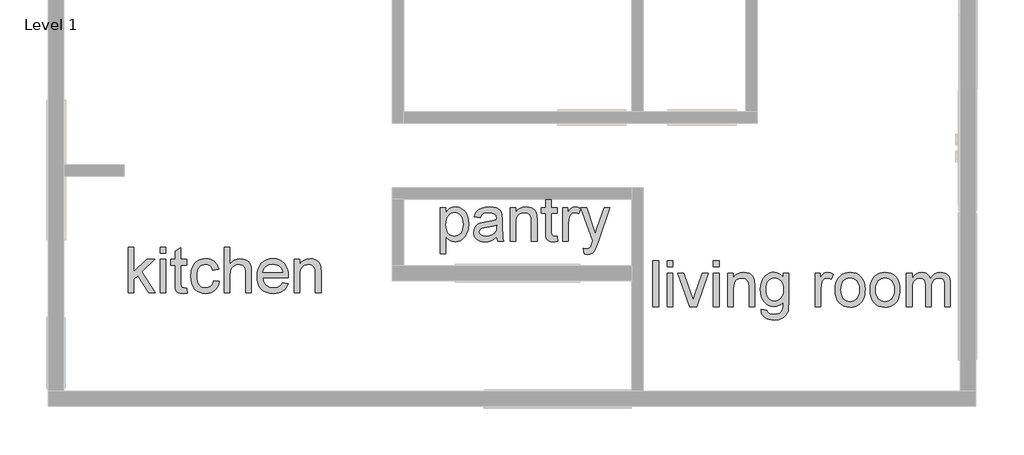
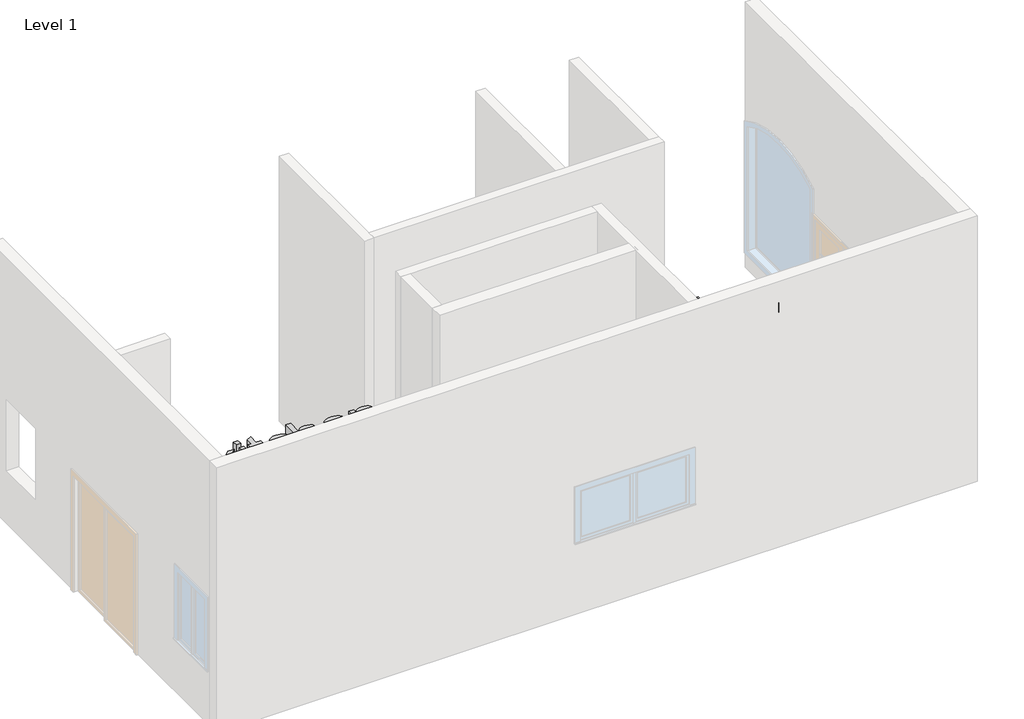
# One storey, part 2 of 3: 3 proxies.
"""IFC4 building model written with IfcOpenShell, lengths in millimetres."""

from ifc_helpers import new_model, si_unit, origin, origin_with_axes, place, context, project, spatial, polyline, outline, extrude, element, save

model = new_model("IFC4")

# Units and contexts
model_context = context("Model", 3, world=origin())
ifc_project = project(units=[si_unit("LENGTHUNIT", "METRE", prefix="MILLI")], contexts=[model_context])

# Site, building, storey
site = spatial("IfcSite", under=ifc_project)
building = spatial("IfcBuilding", under=site)
storey = spatial("IfcBuildingStorey", under=building, Name="Level 1", Elevation=0.0)

# Proxies
placement = place(None, origin())
element("IfcBuildingElementProxy", 1, Name="24\" Arial", ObjectType="24\" Arial", at=placement, inside=storey, context=model_context, shape_type="SweptSolid", body=[
    extrude(outline(polyline([(-77396.9155142, -11295.8130621), (-77396.9155142, -10686.678874), (-77320.7737407, -10686.678874), (-77320.7737407, -11013.9992715), (-77150.0496079, -10848.4801427), (-77044.7598117, -10848.4801427), (-77217.5659461, -11016.0812731), (-77035.24209, -11295.8130621), (-77124.1733021, -11295.8130621), (-77272.1441314, -11069.0236), (-77320.7737407, -11116.1660652), (-77320.7737407, -11295.8130621), (-77396.9155142, -11295.8130621)])), origin_with_axes(), (0.0, 0.0, 1.0), 152.4),
    extrude(outline(polyline([(-76968.6180382, -11295.8130621), (-76968.6180382, -10848.4801427), (-76892.4762647, -10848.4801427), (-76892.4762647, -11295.8130621), (-76968.6180382, -11295.8130621)])), origin_with_axes(), (0.0, 0.0, 1.0), 152.4),
    extrude(outline(polyline([(-76968.6180382, -10762.8206475), (-76968.6180382, -10686.678874), (-76892.4762647, -10686.678874), (-76892.4762647, -10762.8206475), (-76968.6180382, -10762.8206475)])), origin_with_axes(), (0.0, 0.0, 1.0), 152.4),
    extrude(outline(polyline([(-76616.4623357, -11232.3120127), (-76606.944614, -11298.0437781), (-76637.0964589, -11303.5090324), (-76663.9022297, -11305.3307838), (-76700.4487939, -11302.1706028), (-76727.7007079, -11292.6900597), (-76746.9592229, -11278.0788698), (-76759.5255898, -11259.5267482), (-76766.4408095, -11227.6646877), (-76768.7458827, -11173.123681), (-76768.7458827, -10924.6219162), (-76825.8522128, -10924.6219162), (-76825.8522128, -10848.4801427), (-76768.7458827, -10848.4801427), (-76768.7458827, -10739.7699153), (-76692.6041092, -10695.0068805), (-76692.6041092, -10848.4801427), (-76616.4623357, -10848.4801427), (-76616.4623357, -10924.6219162), (-76692.6041092, -10924.6219162), (-76692.6041092, -11170.892965), (-76688.5888204, -11210.1535669), (-76675.5763102, -11224.0583635), (-76664.5900338, -11227.9063486), (-76649.6256472, -11229.1890103), (-76616.4623357, -11232.3120127)])), origin_with_axes(), (0.0, 0.0, 1.0), 152.4),
    extrude(outline(polyline([(-76254.7889115, -11134.0117934), (-76178.6471379, -11143.5295151), (-76186.9286712, -11179.457985), (-76199.8761187, -11211.2503356), (-76217.4894807, -11238.906567), (-76239.7687569, -11262.426679), (-76265.7751879, -11281.1972249), (-76294.5700138, -11294.6047576), (-76326.1532348, -11302.6492773), (-76360.5248509, -11305.3307838), (-76403.2291207, -11301.5896872), (-76441.5184317, -11290.3663972), (-76475.392784, -11271.6609139), (-76504.8521774, -11245.4732373), (-76528.6976022, -11212.2959838), (-76545.7300485, -11172.6217699), (-76555.9495163, -11126.4505956), (-76559.3560055, -11073.7824608), (-76553.5375546, -11006.0244617), (-76546.2644909, -10975.5333621), (-76536.0822017, -10947.3008624), (-76522.9209772, -10921.8939364), (-76506.7111074, -10899.8795577), (-76487.4525925, -10881.2577262), (-76465.1454322, -10866.0284421), (-76440.7980963, -10854.1870579), (-76415.4190543, -10845.7289263), (-76389.0083061, -10840.6540473), (-76361.5658517, -10838.962421), (-76327.7844459, -10841.2860835), (-76297.2282838, -10848.2570711), (-76269.8973652, -10859.8753837), (-76245.7916902, -10876.1410214), (-76225.3202234, -10896.6821981), (-76208.8919293, -10921.1271278), (-76196.5068081, -10949.4758106), (-76188.1648596, -10981.7282464), (-76264.3066332, -10991.2459681), (-76278.1184832, -10958.0268886), (-76299.6263035, -10934.2139951), (-76327.6403789, -10919.8816447), (-76360.9709941, -10915.1041945), (-76386.8426526, -10917.455741), (-76410.1768716, -10924.5103804), (-76430.9736512, -10936.2681128), (-76449.2329913, -10952.7289381), (-76464.0997841, -10974.273937), (-76474.7189218, -11001.2841902), (-76481.0904045, -11033.7596976), (-76483.214232, -11071.7004592), (-76481.1368777, -11110.2128419), (-76474.9048148, -11143.0647826), (-76464.5180434, -11170.2562814), (-76449.9765633, -11191.7873383), (-76432.0797146, -11208.1505698), (-76411.626837, -11219.8385923), (-76388.6179308, -11226.8514058), (-76363.0529957, -11229.1890103), (-76323.62509, -11223.35197), (-76306.5740544, -11216.0556697), (-76291.298297, -11205.8408493), (-76278.2253717, -11192.5959729), (-76267.7828323, -11176.2095048), (-76259.9706789, -11156.681445), (-76254.7889115, -11134.0117934)])), origin_with_axes(), (0.0, 0.0, 1.0), 152.4),
    extrude(outline(polyline([(-76112.0230861, -11295.8130621), (-76112.0230861, -10686.678874), (-76035.8813126, -10686.678874), (-76035.8813126, -10910.6427625), (-76007.9137105, -10879.2826131), (-75976.5070878, -10856.8825064), (-75941.6614447, -10843.4424424), (-75903.376781, -10838.962421), (-75857.3868523, -10843.851407), (-75817.8660002, -10858.5183648), (-75786.7475117, -10881.8107579), (-75775.0641365, -10896.2592915), (-75765.9646741, -10912.5760497), (-75754.253415, -10954.8481183), (-75750.3496619, -11012.6608419), (-75750.3496619, -11295.8130621), (-75826.4914354, -11295.8130621), (-75826.4914354, -11020.5427051), (-75828.0064634, -10994.833703), (-75832.5515473, -10972.8797395), (-75840.1266871, -10954.6808146), (-75850.7318829, -10940.2369284), (-75864.116179, -10929.2413573), (-75880.0286199, -10921.387378), (-75898.4692057, -10916.6749904), (-75919.4379363, -10915.1041945), (-75951.6160149, -10919.342555), (-75981.8236277, -10932.0576363), (-76006.8448257, -10952.0225447), (-76023.4636601, -10978.0103863), (-76032.7768995, -11012.5493061), (-76035.8813126, -11058.1674487), (-76035.8813126, -11295.8130621), (-76112.0230861, -11295.8130621)])), origin_with_axes(), (0.0, 0.0, 1.0), 152.4),
    extrude(outline(polyline([(-75332.462194, -11162.5649585), (-75257.8075645, -11172.0826802), (-75269.2539261, -11201.9835695), (-75284.7062818, -11228.3339025), (-75304.1646318, -11251.1336792), (-75327.6289759, -11270.3828995), (-75354.8576534, -11285.6725989), (-75385.6090032, -11296.5938127), (-75419.8830254, -11303.146541), (-75457.67972, -11305.3307838), (-75504.9244264, -11301.5618032), (-75547.0198966, -11290.2548614), (-75583.9661307, -11271.4099583), (-75615.7631286, -11245.027094), (-75641.332711, -11211.8405459), (-75659.5966985, -11172.5845913), (-75670.5550909, -11127.2592301), (-75674.2078884, -11075.8644625), (-75670.5179123, -11022.7269479), (-75659.4479841, -10975.8912061), (-75640.9981036, -10935.3572371), (-75615.168271, -10901.1250408), (-75583.4549249, -10873.9288947), (-75547.354504, -10854.503076), (-75506.8670082, -10842.8475848), (-75461.9924376, -10838.962421), (-75418.5631851, -10842.8382901), (-75379.2886411, -10854.4658974), (-75344.1688058, -10873.8452428), (-75313.203679, -10900.9763264), (-75287.9268781, -10935.1341655), (-75269.8720203, -10975.5937773), (-75259.0391056, -11022.3551619), (-75255.4281341, -11075.4183193), (-75255.8742773, -11095.9409066), (-75598.0661149, -11095.9409066), (-75593.6558034, -11126.3251178), (-75584.8863011, -11152.935701), (-75571.7576078, -11175.7726562), (-75554.2697237, -11194.8359836), (-75533.3892922, -11209.8654328), (-75510.0829572, -11220.6007536), (-75484.3507184, -11227.0419461), (-75456.1925759, -11229.1890103), (-75415.6679016, -11225.2109001), (-75381.5379464, -11213.2765694), (-75353.8027106, -11192.6424462), (-75332.462194, -11162.5649585)]), holes=[polyline([(-75598.0661149, -11019.7991331), (-75331.5699076, -11019.7991331), (-75341.8683799, -10979.5718875), (-75350.7261814, -10963.7523931), (-75362.0563599, -10950.7956509), (-75382.8206082, -10935.1806387), (-75406.4476087, -10924.0270586), (-75432.9373614, -10917.3349106), (-75462.2898664, -10915.1041945), (-75489.063106, -10916.88412), (-75513.6149242, -10922.2238965), (-75535.945321, -10931.123524), (-75556.0542965, -10943.5830024), (-75572.9287337, -10959.0260635), (-75585.5555159, -10976.876439), (-75593.9346429, -10997.1341289), (-75598.0661149, -11019.7991331)])]), origin_with_axes(), (0.0, 0.0, 1.0), 152.4),
    extrude(outline(polyline([(-75179.2863605, -11295.8130621), (-75179.2863605, -10848.4801427), (-75103.144587, -10848.4801427), (-75103.144587, -10910.9401913), (-75076.6920129, -10879.4499168), (-75044.9228989, -10856.9568636), (-75007.837245, -10843.4610317), (-74965.4350513, -10838.962421), (-74927.9032543, -10842.5873346), (-74893.5316382, -10853.4620752), (-74864.8669374, -10870.2296239), (-74844.4558858, -10891.5329619), (-74830.6068572, -10917.3163213), (-74821.6282252, -10947.523934), (-74817.6129363, -11021.1375627), (-74817.6129363, -11295.8130621), (-74893.7547098, -11295.8130621), (-74893.7547098, -11031.3988564), (-74895.9482473, -10992.0267187), (-74902.5288595, -10964.0312326), (-74914.6676725, -10943.9733777), (-74933.5358122, -10928.4141335), (-74957.7204918, -10918.4316793), (-74985.8089243, -10915.1041945), (-75008.9293664, -10916.9724192), (-75030.4046554, -10922.5770932), (-75050.2347914, -10931.9182166), (-75068.4197743, -10944.9957892), (-75083.6118799, -10963.2969552), (-75094.4633838, -10988.3088586), (-75100.9742862, -11020.0314994), (-75103.144587, -11058.4648775), (-75103.144587, -11295.8130621), (-75179.2863605, -11295.8130621)])), origin_with_axes(), (0.0, 0.0, 1.0), 152.4),
])
element("IfcBuildingElementProxy", 2, Name="24\" Arial", ObjectType="24\" Arial", at=placement, inside=storey, context=model_context, shape_type="SweptSolid", body=[
    extrude(outline(polyline([(-73223.9376122, -10774.6728374), (-73223.9376122, -10156.0209275), (-73147.7958387, -10156.0209275), (-73147.7958387, -10230.675557), (-73122.9605336, -10193.8501534), (-73095.1509406, -10167.5462936), (-73062.7312011, -10151.7639778), (-73024.0654567, -10146.5032058), (-72997.5106414, -10148.3435466), (-72972.5730952, -10153.8645687), (-72949.2528182, -10163.0662723), (-72927.5498102, -10175.9486573), (-72907.9380985, -10192.1771164), (-72890.8917103, -10211.4170421), (-72876.4106454, -10233.6684344), (-72864.494904, -10258.9312933), (-72848.5452845, -10315.0338012), (-72843.2287446, -10376.266956), (-72849.2330886, -10441.3852745), (-72856.7385185, -10471.3651684), (-72867.2461204, -10499.625552), (-72880.6118273, -10525.4275006), (-72896.6915719, -10548.0320896), (-72915.4853544, -10567.439319), (-72936.9931747, -10583.6491888), (-72960.16009, -10596.43398), (-72983.9311576, -10605.5659737), (-73008.3063775, -10611.0451699), (-73033.2857496, -10612.8715686), (-73068.2894018, -10607.9825827), (-73099.5380154, -10593.3156248), (-73126.2880184, -10571.1757683), (-73147.7958387, -10543.8680864), (-73147.7958387, -10774.6728374), (-73223.9376122, -10774.6728374)]), holes=[polyline([(-73147.7958387, -10383.2565329), (-73145.7370737, -10419.9518114), (-73139.5607787, -10451.5164431), (-73129.2669537, -10477.950428), (-73114.8555988, -10499.253766), (-73097.5071344, -10515.6495287), (-73078.4019811, -10527.3607878), (-73057.540139, -10534.3875433), (-73034.921608, -10536.7297951), (-73011.9777643, -10534.3038914), (-72990.7348415, -10527.0261804), (-72971.1928397, -10514.8966621), (-72953.3517588, -10497.9153363), (-72938.484966, -10475.8405424), (-72927.8658283, -10448.4306193), (-72921.4943457, -10415.685567), (-72919.3705181, -10377.6053856), (-72921.4432251, -10341.2261252), (-72927.661346, -10309.7172614), (-72938.0248808, -10283.0787942), (-72952.5338296, -10261.3107237), (-72969.9241199, -10244.3944606), (-72988.9316794, -10232.3114154), (-73009.5565079, -10225.0615884), (-73031.7986056, -10222.6449794), (-73053.9709934, -10225.2149501), (-73074.8328355, -10232.9248624), (-73094.3841319, -10245.7747161), (-73112.6248827, -10263.7645113), (-73128.012176, -10286.6525872), (-73139.0030997, -10314.1972827), (-73145.5976539, -10346.3985979), (-73147.7958387, -10383.2565329)])]), origin_with_axes(), (0.0, 0.0, 1.0), 152.4),
    extrude(outline(polyline([(-72472.0375987, -10546.2475168), (-72508.4168592, -10577.4403625), (-72545.874299, -10597.8514141), (-72585.2650261, -10609.11653), (-72627.4441482, -10612.8715686), (-72661.3463844, -10610.6129687), (-72691.0753227, -10603.8371687), (-72716.6309631, -10592.5441689), (-72738.0133056, -10576.7339691), (-72754.8970375, -10557.4103916), (-72766.956846, -10535.5772585), (-72774.1927311, -10511.2345699), (-72776.6046928, -10484.3823258), (-72772.9611899, -10452.8176941), (-72762.0306814, -10424.1529933), (-72745.1701862, -10399.615117), (-72723.7367231, -10380.4309592), (-72698.5482213, -10365.9313051), (-72670.4226102, -10355.4469398), (-72604.5421304, -10343.9959309), (-72526.6901412, -10331.9500644), (-72472.4837419, -10317.8221963), (-72472.0375987, -10300.8687545), (-72477.2797814, -10266.8875138), (-72483.8325097, -10254.3025576), (-72493.0063293, -10244.6547108), (-72508.8630024, -10235.0254533), (-72528.1772852, -10228.1474122), (-72577.1786805, -10222.6449794), (-72622.5365729, -10226.3070715), (-72654.2127404, -10237.2933479), (-72675.8135072, -10257.611453), (-72690.9451976, -10289.2690312), (-72767.0869711, -10279.7513095), (-72753.8699787, -10238.1112771), (-72734.1467312, -10205.3941088), (-72706.0768879, -10180.3729108), (-72667.8201082, -10161.8207892), (-72621.0308396, -10150.3326017), (-72567.36353, -10146.5032058), (-72515.8897578, -10149.8864585), (-72475.0862439, -10160.0362164), (-72444.3209521, -10175.2980318), (-72422.9618462, -10194.0174571), (-72408.7967995, -10217.1611358), (-72399.6136852, -10245.6957116), (-72395.8958252, -10312.3197634), (-72395.8958252, -10407.0508371), (-72392.0292508, -10539.3322971), (-72386.3037463, -10572.0308761), (-72376.8603818, -10603.3538469), (-72453.0021553, -10603.3538469), (-72465.1967362, -10576.8826835), (-72472.0375987, -10546.2475168)]), holes=[polyline([(-72472.0375987, -10393.9639698), (-72523.1953528, -10406.6418725), (-72594.8756943, -10417.3121308), (-72660.3843881, -10429.6554261), (-72677.4307763, -10438.0949684), (-72690.0529112, -10449.7318703), (-72697.8604172, -10463.6738454), (-72700.4629193, -10479.0286074), (-72694.7931827, -10501.670375), (-72677.783973, -10520.2224966), (-72649.8070763, -10532.6029705), (-72611.2342784, -10536.7297951), (-72570.337818, -10532.1754166), (-72534.2002185, -10518.5122809), (-72504.9034814, -10498.3800689), (-72484.5296084, -10474.4184609), (-72475.4952085, -10449.7318703), (-72472.4837419, -10415.527558), (-72472.0375987, -10393.9639698)])]), origin_with_axes(), (0.0, 0.0, 1.0), 152.4),
    extrude(outline(polyline([(-72291.2008866, -10603.3538469), (-72291.2008866, -10156.0209275), (-72215.0591131, -10156.0209275), (-72215.0591131, -10218.4809761), (-72188.6065389, -10186.9907016), (-72156.8374249, -10164.4976484), (-72119.7517711, -10151.0018165), (-72077.3495774, -10146.5032058), (-72039.8177803, -10150.1281194), (-72005.4461643, -10161.00286), (-71976.7814634, -10177.7704087), (-71956.3704119, -10199.0737467), (-71942.5213832, -10224.8571061), (-71933.5427512, -10255.0647189), (-71929.5274624, -10328.6783476), (-71929.5274624, -10603.3538469), (-72005.6692359, -10603.3538469), (-72005.6692359, -10338.9396413), (-72007.8627733, -10299.5675035), (-72014.4433856, -10271.5720174), (-72026.5821986, -10251.5141625), (-72045.4503383, -10235.9549183), (-72069.6350178, -10225.9724641), (-72097.7234504, -10222.6449794), (-72120.8438925, -10224.513204), (-72142.3191815, -10230.117878), (-72162.1493175, -10239.4590014), (-72180.3343004, -10252.536574), (-72195.5264059, -10270.8377401), (-72206.3779099, -10295.8496434), (-72212.8888123, -10327.5722842), (-72215.0591131, -10366.0056623), (-72215.0591131, -10603.3538469), (-72291.2008866, -10603.3538469)])), origin_with_axes(), (0.0, 0.0, 1.0), 152.4),
    extrude(outline(polyline([(-71663.0312551, -10539.8527975), (-71653.5135334, -10605.584563), (-71683.6653783, -10611.0498172), (-71710.4711491, -10612.8715686), (-71747.0177133, -10609.7113876), (-71774.2696273, -10600.2308445), (-71793.5281423, -10585.6196546), (-71806.0945092, -10567.067533), (-71813.0097289, -10535.2054725), (-71815.3148021, -10480.6644658), (-71815.3148021, -10232.162701), (-71872.4211323, -10232.162701), (-71872.4211323, -10156.0209275), (-71815.3148021, -10156.0209275), (-71815.3148021, -10047.3107001), (-71739.1730286, -10002.5476653), (-71739.1730286, -10156.0209275), (-71663.0312551, -10156.0209275), (-71663.0312551, -10232.162701), (-71739.1730286, -10232.162701), (-71739.1730286, -10478.4337498), (-71735.1577398, -10517.6943517), (-71722.1452296, -10531.5991483), (-71711.1589532, -10535.4471334), (-71696.1945666, -10536.7297951), (-71663.0312551, -10539.8527975)])), origin_with_axes(), (0.0, 0.0, 1.0), 152.4),
    extrude(outline(polyline([(-71586.8894816, -10603.3538469), (-71586.8894816, -10156.0209275), (-71520.2654297, -10156.0209275), (-71520.2654297, -10222.1988362), (-71495.6531963, -10183.8305206), (-71472.9742501, -10161.2259316), (-71450.2209467, -10150.1838873), (-71425.3856417, -10146.5032058), (-71387.4634693, -10152.3774247), (-71348.9464393, -10170.0000813), (-71374.376602, -10238.2599915), (-71401.1451942, -10226.5487324), (-71427.9137865, -10222.6449794), (-71450.6485006, -10226.400018), (-71470.9666057, -10237.6651339), (-71487.3809577, -10255.5852193), (-71498.4044127, -10279.3051663), (-71507.6618842, -10321.8374851), (-71510.7477081, -10368.2363783), (-71510.7477081, -10603.3538469), (-71586.8894816, -10603.3538469)])), origin_with_axes(), (0.0, 0.0, 1.0), 152.4),
    extrude(outline(polyline([(-71301.3578309, -10774.6728374), (-71310.8755526, -10701.3566375), (-71272.2098082, -10708.0487855), (-71251.8731138, -10705.9481946), (-71236.0722087, -10699.6464218), (-71223.766092, -10689.5896105), (-71213.9137629, -10676.2239036), (-71193.0937467, -10620.1585743), (-71187.1451706, -10601.7179885), (-71348.9464393, -10156.0209275), (-71268.6406626, -10156.0209275), (-71182.832453, -10404.3739779), (-71152.9408583, -10503.715198), (-71123.0492636, -10415.9737012), (-71034.8616236, -10156.0209275), (-70955.1507044, -10156.0209275), (-71110.8546827, -10614.0612838), (-71151.3049999, -10713.402504), (-71172.0134803, -10745.1158501), (-71195.4731771, -10767.0884029), (-71222.7250911, -10779.91502), (-71254.8102232, -10784.190559), (-71276.8571333, -10781.8111286), (-71301.3578309, -10774.6728374)])), origin_with_axes(), (0.0, 0.0, 1.0), 152.4),
])
element("IfcBuildingElementProxy", 3, Name="24\" Arial", ObjectType="24\" Arial", at=placement, inside=storey, context=model_context, shape_type="SweptSolid", body=[
    extrude(outline(polyline([(-70381.2103077, -11478.0391714), (-70381.2103077, -10868.9049832), (-70305.0685342, -10868.9049832), (-70305.0685342, -11478.0391714), (-70381.2103077, -11478.0391714)])), origin_with_axes(), (0.0, 0.0, 1.0), 152.4),
    extrude(outline(polyline([(-70190.855874, -11478.0391714), (-70190.855874, -11030.706252), (-70114.7141004, -11030.706252), (-70114.7141004, -11478.0391714), (-70190.855874, -11478.0391714)])), origin_with_axes(), (0.0, 0.0, 1.0), 152.4),
    extrude(outline(polyline([(-70190.855874, -10945.0467568), (-70190.855874, -10868.9049832), (-70114.7141004, -10868.9049832), (-70114.7141004, -10945.0467568), (-70190.855874, -10945.0467568)])), origin_with_axes(), (0.0, 0.0, 1.0), 152.4),
    extrude(outline(polyline([(-69890.7502119, -11478.0391714), (-70048.0900486, -11030.706252), (-69967.4868431, -11030.706252), (-69872.1609118, -11298.6896033), (-69843.4590323, -11388.8105305), (-69815.3520104, -11303.7458929), (-69719.4312215, -11030.706252), (-69638.828016, -11030.706252), (-69794.2345654, -11478.0391714), (-69890.7502119, -11478.0391714)])), origin_with_axes(), (0.0, 0.0, 1.0), 152.4),
    extrude(outline(polyline([(-69572.2039641, -11478.0391714), (-69572.2039641, -11030.706252), (-69496.0621906, -11030.706252), (-69496.0621906, -11478.0391714), (-69572.2039641, -11478.0391714)])), origin_with_axes(), (0.0, 0.0, 1.0), 152.4),
    extrude(outline(polyline([(-69572.2039641, -10945.0467568), (-69572.2039641, -10868.9049832), (-69496.0621906, -10868.9049832), (-69496.0621906, -10945.0467568), (-69572.2039641, -10945.0467568)])), origin_with_axes(), (0.0, 0.0, 1.0), 152.4),
    extrude(outline(polyline([(-69381.8495303, -11478.0391714), (-69381.8495303, -11030.706252), (-69305.7077568, -11030.706252), (-69305.7077568, -11093.1663006), (-69279.2551827, -11061.6760261), (-69247.4860687, -11039.1829729), (-69210.4004148, -11025.6871409), (-69167.9982211, -11021.1885303), (-69130.4664241, -11024.8134438), (-69096.094808, -11035.6881844), (-69067.4301072, -11052.4557332), (-69047.0190556, -11073.7590712), (-69033.170027, -11099.5424305), (-69024.191395, -11129.7500433), (-69020.1761061, -11203.363672), (-69020.1761061, -11478.0391714), (-69096.3178796, -11478.0391714), (-69096.3178796, -11213.6249657), (-69098.5114171, -11174.2528279), (-69105.0920293, -11146.2573419), (-69117.2308423, -11126.199487), (-69136.098982, -11110.6402427), (-69160.2836616, -11100.6577885), (-69188.3720941, -11097.3303038), (-69211.4925362, -11099.1985285), (-69232.9678252, -11104.8032025), (-69252.7979612, -11114.1443258), (-69270.9829441, -11127.2218985), (-69286.1750497, -11145.5230645), (-69297.0265536, -11170.5349679), (-69303.537456, -11202.2576086), (-69305.7077568, -11240.6909868), (-69305.7077568, -11478.0391714), (-69381.8495303, -11478.0391714)])), origin_with_axes(), (0.0, 0.0, 1.0), 152.4),
    extrude(outline(polyline([(-68934.5166109, -11516.1100581), (-68858.3748374, -11525.6277798), (-68849.9724737, -11549.4220841), (-68833.6882468, -11565.7806682), (-68801.6774719, -11578.4957495), (-68759.7771893, -11582.73411), (-68715.0885117, -11577.9380705), (-68697.0383012, -11571.9430212), (-68681.8508429, -11563.5499522), (-68658.8001107, -11540.49922), (-68644.6722426, -11509.7153389), (-68640.545418, -11476.960992), (-68639.4672385, -11420.9328412), (-68664.8044547, -11445.9168607), (-68693.0787803, -11463.7625889), (-68724.2902152, -11474.4700258), (-68758.4387597, -11478.0391714), (-68800.1856805, -11473.8844628), (-68836.9413743, -11461.420337), (-68868.705841, -11440.6467941), (-68895.4790806, -11411.563834), (-68916.7220033, -11376.6717175), (-68931.8955196, -11338.4707057), (-68940.9996294, -11296.9607984), (-68944.0343326, -11252.1419957), (-68938.5876677, -11190.66718), (-68922.2476728, -11134.1371181), (-68910.1367437, -11108.6465403), (-68895.5906164, -11086.2324916), (-68878.6092906, -11066.8949721), (-68859.1927666, -11050.6339818), (-68837.652415, -11037.7515967), (-68814.2996067, -11028.5498932), (-68789.1343416, -11023.028871), (-68762.1566197, -11021.1885303), (-68726.5488152, -11025.3525335), (-68694.2313169, -11037.8445432), (-68665.2041246, -11058.6645594), (-68639.4672385, -11087.8125821), (-68639.4672385, -11030.706252), (-68563.325465, -11030.706252), (-68563.325465, -11416.9175524), (-68568.5304691, -11506.0904254), (-68575.0367241, -11539.2583842), (-68584.1454812, -11564.8140246), (-68596.0751646, -11585.4249112), (-68611.0441986, -11603.7586085), (-68629.0525831, -11619.8151165), (-68650.1003182, -11633.5944353), (-68673.973627, -11644.6550689), (-68700.4587324, -11652.5555214), (-68729.5556345, -11657.295793), (-68761.2643333, -11658.8758835), (-68798.5684114, -11656.6498148), (-68832.1081563, -11649.9716087), (-68861.8835678, -11638.8412652), (-68887.8946461, -11623.2587844), (-68908.9052026, -11603.2055768), (-68923.6790489, -11578.6630532), (-68932.216185, -11549.6312137), (-68934.5166109, -11516.1100581)]), holes=[polyline([(-68867.8925591, -11246.9369916), (-68865.8616781, -11284.5849718), (-68859.7690349, -11316.7769924), (-68849.6146297, -11343.5130533), (-68835.3984624, -11364.7931547), (-68818.1150606, -11381.0262611), (-68798.7589517, -11392.6213371), (-68777.330136, -11399.5783827), (-68753.8286132, -11401.8973979), (-68730.5594567, -11399.5923246), (-68709.2328821, -11392.677105), (-68689.8488893, -11381.1517389), (-68672.4074785, -11365.0162263), (-68657.9961235, -11343.9452546), (-68647.7022985, -11317.6135109), (-68641.5260035, -11286.0209952), (-68639.4672385, -11249.1677076), (-68641.5864188, -11213.8526846), (-68647.9439594, -11183.1571027), (-68658.5398605, -11157.0809619), (-68673.3741221, -11135.6242622), (-68691.1919663, -11118.8706554), (-68710.7386154, -11106.9037934), (-68732.0140695, -11099.7236762), (-68755.0183284, -11097.3303038), (-68777.6368594, -11099.6864976), (-68798.4987015, -11106.755079), (-68817.6038548, -11118.536048), (-68834.9523192, -11135.0294046), (-68849.3636741, -11156.1607915), (-68859.6574991, -11181.8558517), (-68865.8337941, -11212.1145851), (-68867.8925591, -11246.9369916)])]), origin_with_axes(), (0.0, 0.0, 1.0), 152.4),
    extrude(outline(polyline([(-68211.1697625, -11478.0391714), (-68211.1697625, -11030.706252), (-68144.5457107, -11030.706252), (-68144.5457107, -11096.8841606), (-68119.9334773, -11058.515845), (-68097.254531, -11035.911256), (-68074.5012276, -11024.8692117), (-68049.6659226, -11021.1885303), (-68011.7437502, -11027.0627491), (-67973.2267203, -11044.6854057), (-67998.6568829, -11112.9453159), (-68025.4254752, -11101.2340568), (-68052.1940674, -11097.3303038), (-68074.9287815, -11101.0853424), (-68095.2468866, -11112.3504583), (-68111.6612387, -11130.2705437), (-68122.6846937, -11153.9904907), (-68131.9421652, -11196.5228095), (-68135.027989, -11242.9217028), (-68135.027989, -11478.0391714), (-68211.1697625, -11478.0391714)])), origin_with_axes(), (0.0, 0.0, 1.0), 152.4),
    extrude(outline(polyline([(-67944.6735552, -11254.3727117), (-67940.5560252, -11196.4391577), (-67928.2034352, -11146.5175921), (-67907.6157853, -11104.6080148), (-67878.7930754, -11070.710426), (-67849.7751778, -11049.0445966), (-67817.7458136, -11033.5690042), (-67782.7049828, -11024.2836488), (-67744.6526853, -11021.1885303), (-67702.6455142, -11024.9575109), (-67664.6629267, -11036.2644527), (-67630.7049226, -11055.1093558), (-67600.771502, -11081.4922201), (-67576.3405142, -11114.5207591), (-67558.8898087, -11153.3026866), (-67548.4193853, -11197.8380025), (-67544.9292442, -11248.1267068), (-67546.4721562, -11288.8837475), (-67551.1008919, -11325.0492309), (-67558.8154515, -11356.6231573), (-67569.6158349, -11383.6055265), (-67583.3672697, -11406.9118616), (-67599.9349835, -11427.4576856), (-67619.3189762, -11445.2429986), (-67641.5192479, -11460.2678004), (-67665.6713962, -11472.2067785), (-67690.9110185, -11480.7346199), (-67717.2381149, -11485.8513248), (-67744.6526853, -11487.5568931), (-67787.2733033, -11483.8018544), (-67825.6090876, -11472.5367385), (-67859.6600382, -11453.7615454), (-67889.4261551, -11427.4762749), (-67913.5968926, -11394.1270704), (-67930.8617052, -11354.160075), (-67941.2205927, -11307.5752888), (-67944.6735552, -11254.3727117)]), holes=[polyline([(-67868.5317817, -11254.2239973), (-67866.3289496, -11291.1562894), (-67859.7204534, -11323.134533), (-67848.706293, -11350.1587282), (-67833.2864686, -11372.2288748), (-67814.5298647, -11389.3728569), (-67793.5053662, -11401.6185584), (-67770.2129731, -11408.9659793), (-67744.6526853, -11411.4151196), (-67719.2225227, -11408.9520373), (-67696.0230761, -11401.5627905), (-67675.0543455, -11389.2473791), (-67656.3163309, -11372.0058032), (-67640.8965064, -11349.7172323), (-67629.882346, -11322.2608359), (-67623.2738498, -11289.6366141), (-67621.0710178, -11251.8445669), (-67623.2877918, -11216.0834006), (-67629.9381139, -11184.9416755), (-67641.0219842, -11158.4193915), (-67656.5394025, -11136.5165486), (-67675.3471269, -11119.3725665), (-67696.3019156, -11107.126865), (-67719.4037684, -11099.7794441), (-67744.6526853, -11097.3303038), (-67770.2129731, -11099.7701494), (-67793.5053662, -11107.0896864), (-67814.5298647, -11119.2889146), (-67833.2864686, -11136.3678342), (-67848.706293, -11158.3729183), (-67859.7204534, -11185.3506401), (-67866.3289496, -11217.3009998), (-67868.5317817, -11254.2239973)])]), origin_with_axes(), (0.0, 0.0, 1.0), 152.4),
    extrude(outline(polyline([(-67478.3051924, -11254.3727117), (-67474.1876624, -11196.4391577), (-67461.8350725, -11146.5175921), (-67441.2474225, -11104.6080148), (-67412.4247126, -11070.710426), (-67383.406815, -11049.0445966), (-67351.3774508, -11033.5690042), (-67316.33662, -11024.2836488), (-67278.2843225, -11021.1885303), (-67236.2771515, -11024.9575109), (-67198.2945639, -11036.2644527), (-67164.3365598, -11055.1093558), (-67134.4031392, -11081.4922201), (-67109.9721514, -11114.5207591), (-67092.5214459, -11153.3026866), (-67082.0510226, -11197.8380025), (-67078.5608814, -11248.1267068), (-67080.1037934, -11288.8837475), (-67084.7325291, -11325.0492309), (-67092.4470887, -11356.6231573), (-67103.2474721, -11383.6055265), (-67116.9989069, -11406.9118616), (-67133.5666207, -11427.4576856), (-67152.9506134, -11445.2429986), (-67175.1508852, -11460.2678004), (-67199.3030334, -11472.2067785), (-67224.5426557, -11480.7346199), (-67250.8697521, -11485.8513248), (-67278.2843225, -11487.5568931), (-67320.9049405, -11483.8018544), (-67359.2407248, -11472.5367385), (-67393.2916754, -11453.7615454), (-67423.0577923, -11427.4762749), (-67447.2285298, -11394.1270704), (-67464.4933424, -11354.160075), (-67474.8522299, -11307.5752888), (-67478.3051924, -11254.3727117)]), holes=[polyline([(-67402.1634189, -11254.2239973), (-67399.9605868, -11291.1562894), (-67393.3520906, -11323.134533), (-67382.3379303, -11350.1587282), (-67366.9181058, -11372.2288748), (-67348.1615019, -11389.3728569), (-67327.1370034, -11401.6185584), (-67303.8446103, -11408.9659793), (-67278.2843225, -11411.4151196), (-67252.8541599, -11408.9520373), (-67229.6547133, -11401.5627905), (-67208.6859827, -11389.2473791), (-67189.9479681, -11372.0058032), (-67174.5281436, -11349.7172323), (-67163.5139832, -11322.2608359), (-67156.905487, -11289.6366141), (-67154.702655, -11251.8445669), (-67156.919429, -11216.0834006), (-67163.5697511, -11184.9416755), (-67174.6536214, -11158.4193915), (-67190.1710397, -11136.5165486), (-67208.9787641, -11119.3725665), (-67229.9335528, -11107.126865), (-67253.0354056, -11099.7794441), (-67278.2843225, -11097.3303038), (-67303.8446103, -11099.7701494), (-67327.1370034, -11107.0896864), (-67348.1615019, -11119.2889146), (-67366.9181058, -11136.3678342), (-67382.3379303, -11158.3729183), (-67393.3520906, -11185.3506401), (-67399.9605868, -11217.3009998), (-67402.1634189, -11254.2239973)])]), origin_with_axes(), (0.0, 0.0, 1.0), 152.4),
    extrude(outline(polyline([(-66992.9013862, -11478.0391714), (-66992.9013862, -11030.706252), (-66916.7596127, -11030.706252), (-66916.7596127, -11104.3198807), (-66893.8575949, -11070.5059436), (-66864.4121434, -11044.0161909), (-66829.4270805, -11026.8954454), (-66789.9062283, -11021.1885303), (-66747.5598025, -11027.0069812), (-66729.537476, -11034.2800449), (-66713.6157404, -11044.4623341), (-66699.841069, -11057.2657146), (-66688.259935, -11072.4020523), (-66671.6782792, -11109.6735991), (-66643.9244541, -11070.9613815), (-66612.2668759, -11043.3097975), (-66576.7055446, -11026.7188471), (-66537.2404603, -11021.1885303), (-66506.7586554, -11023.4889562), (-66480.0040051, -11030.3902339), (-66456.9765095, -11041.8923634), (-66437.6761686, -11057.9953446), (-66422.4190005, -11078.8850707), (-66411.5210233, -11104.7474346), (-66404.9822369, -11135.5824362), (-66402.8026415, -11171.3900757), (-66402.8026415, -11478.0391714), (-66478.944415, -11478.0391714), (-66478.944415, -11204.107244), (-66480.7103985, -11166.1293037), (-66486.0083491, -11140.5318374), (-66495.9350354, -11123.0021273), (-66511.5872261, -11109.2274559), (-66531.7194382, -11100.3045918), (-66555.0861885, -11097.3303038), (-66576.6637187, -11099.2357071), (-66596.3358456, -11104.9519169), (-66614.1025692, -11114.4789332), (-66629.9638896, -11127.8167561), (-66643.008931, -11145.3557608), (-66652.3268177, -11167.4863227), (-66657.9175498, -11194.2084417), (-66659.7811271, -11225.5221178), (-66659.7811271, -11478.0391714), (-66735.9229006, -11478.0391714), (-66735.9229006, -11195.6305231), (-66740.3285648, -11152.5777039), (-66745.8356449, -11135.6800301), (-66753.5455572, -11121.86818), (-66763.765025, -11111.1328592), (-66776.8007717, -11103.4647729), (-66792.6527974, -11098.8639211), (-66811.3211021, -11097.3303038), (-66840.6550178, -11101.4199498), (-66867.6838603, -11113.688888), (-66889.9910205, -11133.8396893), (-66905.1598894, -11161.5749252), (-66913.8596819, -11200.0547766), (-66916.7596127, -11252.4394245), (-66916.7596127, -11478.0391714), (-66992.9013862, -11478.0391714)])), origin_with_axes(), (0.0, 0.0, 1.0), 152.4),
])

save(model, "model.ifc")

# Revit data of these elements
# Project information
#   Project Issue Date = "Issue Date"
#   Project Status = "Project Status"
#   Client Name = "Owner"
#   Project Address = "Enter address here"
#   Project Name = "Project Name"
#   Project Number = "Project Number"
# Elements 1, 2, 3 (IfcBuildingElementProxy, "24\" Arial")
#   Phase Created = New Construction
